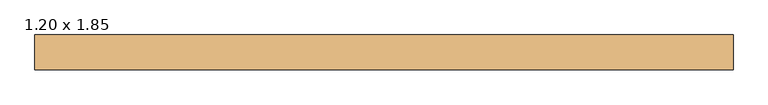
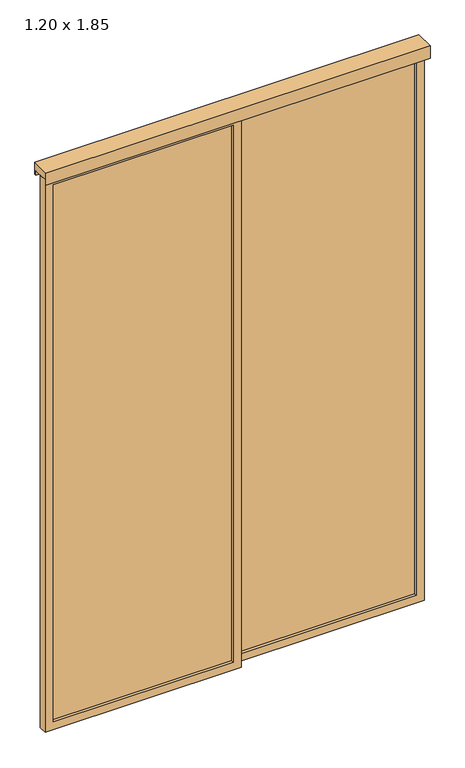
"""IFC4 building model written with IfcOpenShell, lengths in millimetres: door geometry, CC_ND-200_BOX-BANHEIRO : 1.20 x 1.85."""

from ifc_helpers import new_model, si_unit, frame, origin, place, context, project, spatial, polyline, outline, extrude, faceted_brep, source, transform, mapped, element, save


def door_1_20_x_1_85_7a0dc905(model_context):
    return source(origin(), model_context, "Body", "SolidModel", [
        extrude(outline(polyline([(602.5, 15.0), (602.5, 10.0), (10.0, 10.0), (10.0, 15.0), (602.5, 15.0)])), frame((0.0, 0.0, 10.0), z_axis=(0.0, 0.0, 1.0), x_axis=(1.0, 0.0, 0.0)), (0.0, 0.0, 1.0), 1805.0),
        faceted_brep([(587.5, 15.0, 1800.0), (587.5, 25.0, 1800.0), (587.5, 25.0, 25.0), (587.5, 15.0, 25.0), (612.5, 25.0, 1825.0), (612.5, 25.0, 0.0), (0.0, 25.0, 0.0), (0.0, 25.0, 1825.0), (25.0, 25.0, 1800.0), (25.0, 25.0, 25.0), (25.0, 15.0, 25.0), (10.0, 15.0, 1815.0), (10.0, 15.0, 10.0), (602.5, 15.0, 10.0), (602.5, 15.0, 1815.0), (25.0, 15.0, 1800.0), (612.5, 0.0, 1825.0), (612.5, 0.0, 0.0), (0.0, 0.0, 1825.0), (0.0, 0.0, 0.0), (587.5, 0.0, 1800.0), (587.5, 0.0, 25.0), (25.0, 0.0, 25.0), (25.0, 0.0, 1800.0), (587.5, 10.0, 1800.0), (587.5, 10.0, 25.0), (25.0, 10.0, 25.0), (25.0, 10.0, 1800.0), (602.5, 10.0, 1815.0), (602.5, 10.0, 10.0), (10.0, 10.0, 10.0), (10.0, 10.0, 1815.0)], [[[0, 1, 2, 3]], [[4, 5, 6, 7], [8, 9, 2, 1]], [[3, 2, 9, 10]], [[11, 12, 13, 14], [0, 3, 10, 15]], [[4, 16, 17, 5]], [[18, 19, 17, 16], [20, 21, 22, 23]], [[5, 17, 19, 6]], [[10, 9, 8, 15]], [[6, 19, 18, 7]], [[20, 24, 25, 21]], [[21, 25, 26, 22]], [[22, 26, 27, 23]], [[28, 14, 13, 29]], [[29, 13, 12, 30]], [[28, 29, 30, 31], [27, 26, 25, 24]], [[30, 12, 11, 31]], [[15, 8, 1, 0]], [[7, 18, 16, 4]], [[31, 11, 14, 28]], [[23, 27, 24, 20]]]),
        extrude(outline(polyline([(1190.0, 40.0), (1190.0, 35.0), (597.5, 35.0), (597.5, 40.0), (1190.0, 40.0)])), frame((0.0, 0.0, 10.0), z_axis=(0.0, 0.0, 1.0), x_axis=(1.0, 0.0, 0.0)), (0.0, 0.0, 1.0), 1805.0),
        faceted_brep([(1175.0, 40.0, 1800.0), (1175.0, 50.0, 1800.0), (1175.0, 50.0, 25.0), (1175.0, 40.0, 25.0), (1200.0, 50.0, 1825.0), (1200.0, 50.0, 0.0), (587.5, 50.0, 0.0), (587.5, 50.0, 1825.0), (612.5, 50.0, 1800.0), (612.5, 50.0, 25.0), (612.5, 40.0, 25.0), (597.5, 40.0, 1815.0), (597.5, 40.0, 10.0), (1190.0, 40.0, 10.0), (1190.0, 40.0, 1815.0), (612.5, 40.0, 1800.0), (1200.0, 25.0, 1825.0), (1200.0, 25.0, 0.0), (587.5, 25.0, 1825.0), (587.5, 25.0, 0.0), (1175.0, 25.0, 1800.0), (1175.0, 25.0, 25.0), (612.5, 25.0, 25.0), (612.5, 25.0, 1800.0), (1175.0, 35.0, 1800.0), (1175.0, 35.0, 25.0), (612.5, 35.0, 25.0), (612.5, 35.0, 1800.0), (1190.0, 35.0, 1815.0), (1190.0, 35.0, 10.0), (597.5, 35.0, 10.0), (597.5, 35.0, 1815.0)], [[[0, 1, 2, 3]], [[4, 5, 6, 7], [8, 9, 2, 1]], [[3, 2, 9, 10]], [[11, 12, 13, 14], [0, 3, 10, 15]], [[4, 16, 17, 5]], [[18, 19, 17, 16], [20, 21, 22, 23]], [[5, 17, 19, 6]], [[10, 9, 8, 15]], [[6, 19, 18, 7]], [[20, 24, 25, 21]], [[21, 25, 26, 22]], [[22, 26, 27, 23]], [[28, 14, 13, 29]], [[29, 13, 12, 30]], [[28, 29, 30, 31], [27, 26, 25, 24]], [[30, 12, 11, 31]], [[15, 8, 1, 0]], [[7, 18, 16, 4]], [[31, 11, 14, 28]], [[23, 27, 24, 20]]]),
        extrude(outline(polyline([(-5.0, 1810.0), (-5.0, 1850.0), (55.0, 1850.0), (55.0, 1810.0), (50.0, 1810.0), (50.0, 1825.0), (0.0, 1825.0), (0.0, 1810.0), (-5.0, 1810.0)])), frame((0.0, 0.0, 0.0), z_axis=(1.0, 0.0, 0.0), x_axis=(0.0, 1.0, 0.0)), (0.0, 0.0, 1.0), 1200.0),
    ])


if __name__ == "__main__":
    model = new_model("IFC4")
    model_context = context("Model", 3, world=origin())
    ifc_project = project(units=[si_unit("LENGTHUNIT", "METRE", prefix="MILLI")], contexts=[model_context])
    site = spatial("IfcSite", under=ifc_project)
    building = spatial("IfcBuilding", under=site)
    placement = place(None, origin())
    door_1_20_x_1_85_shape = door_1_20_x_1_85_7a0dc905(model_context)
    element("IfcDoor", 1, ObjectType="CC_ND-200_BOX-BANHEIRO : 1.20 x 1.85", at=placement, inside=building, context=model_context, shape_type="MappedRepresentation", body=[
        mapped(door_1_20_x_1_85_shape, transform((0.0, 0.0, 0.0), x_axis=(1.0, 0.0, 0.0), y_axis=(0.0, 1.0, 0.0), z_axis=(0.0, 0.0, 1.0))),
    ])
    save(model, "model.ifc")

# Revit data of these elements
# Type "CC_ND-200_BOX-BANHEIRO : 1.20 x 1.85"
#   Type Mark = "145"
#   Width = 1.20 m
#   Material montante = Aluminio
#   Materia vidro = Vidro
# Element 1 (IfcDoor, "CC_ND-200_BOX-BANHEIRO : 1.20 x 1.85")
#   Materials on its faces: "Aluminio", "Vidro"
# Materials
#   "Aluminio": class "Genérico", colour RGB 120 120 120, transparency 0, Cost = 0
#   "Vidro": class "Vidro", colour RGB 230 230 230, transparency 0.75, Description = "JANELA COM 04 FOLHAS DE CORRER E VIDRO TRANSPARENTE 6mm", Cost = 0
